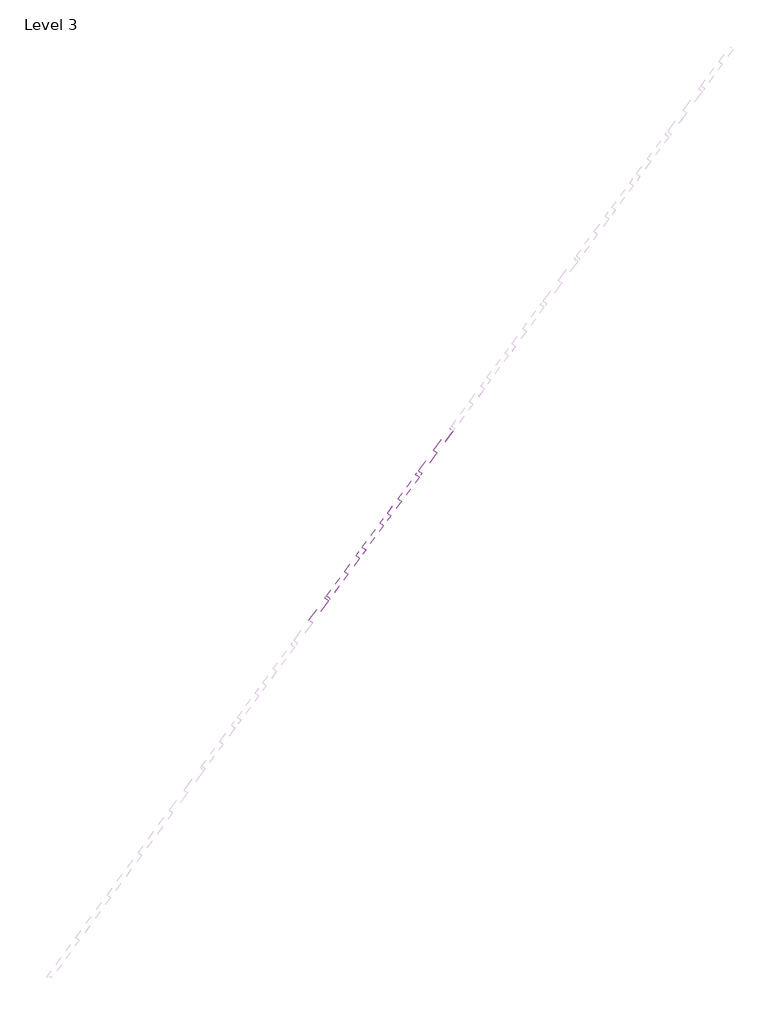
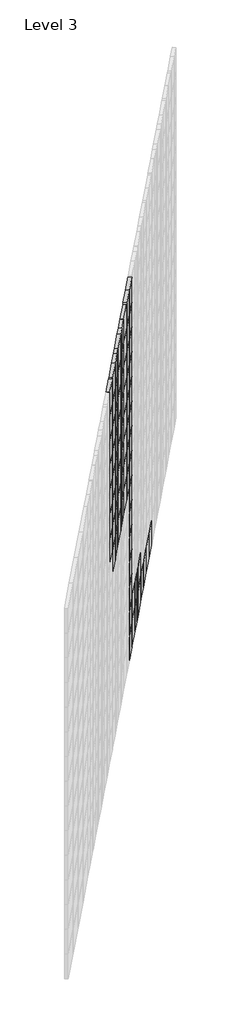
# One storey, part 6 of 9: 117 plates.
"""IFC4 building model written with IfcOpenShell, lengths in millimetres."""

import ifcopenshell
import ifcopenshell.guid

model = None  # the IFC model being written
_history = None  # IfcOwnerHistory: only IFC2X3 demands one
_inside = {}  # id of a spatial element -> (the spatial element, [elements in it])
_under = {}  # id of a project, library or spatial element -> (it, [spatial elements below it])
_declared = {}  # id of a project -> (the project, [libraries it declares])
_typed = {}  # id of a type object -> (the type object, [elements of that type])
_made_of = {}  # id of a material, layer set ... -> (it, [elements and type objects made of it])


def new_model(schema):
    """Start an empty IFC model of exactly this schema.

    Asked for "IFC4X3", IfcOpenShell would pick the latest addendum, in which some entities
    have other attributes; the version numbers below select the first issue.
    IFC2X3 requires an IfcOwnerHistory on every rooted entity: one is made here for all.
    """
    global model, _history
    if schema == "IFC4X3":
        model = ifcopenshell.file(schema_version=(4, 3, 0, 0))
    else:
        model = ifcopenshell.file(schema=schema)
    _inside.clear()
    _under.clear()
    _declared.clear()
    _typed.clear()
    _made_of.clear()
    _history = None
    if model.schema == "IFC2X3":
        org = make("IfcOrganization", Name="unknown")
        user = make(
            "IfcPersonAndOrganization",
            ThePerson=make("IfcPerson", FamilyName="unknown"),
            TheOrganization=org,
        )
        app = make(
            "IfcApplication",
            ApplicationDeveloper=org,
            Version="unknown",
            ApplicationFullName="unknown",
            ApplicationIdentifier="unknown",
        )
        _history = make(
            "IfcOwnerHistory",
            OwningUser=user,
            OwningApplication=app,
            ChangeAction="ADDED",
            CreationDate=0,
        )
    return model


def make(cls, **values):
    """One entity of the class cls with the attributes given. An attribute that is None is left unset."""
    return model.create_entity(
        cls, **{name: value for name, value in values.items() if value is not None}
    )


def rooted(cls, **values):
    """An entity with a GlobalId (a new one), such as an element, a storey or a relation."""
    return make(cls, GlobalId=ifcopenshell.guid.new(), OwnerHistory=_history, **values)


def si_unit(unit_type, name, prefix=None):
    """IfcSIUnit, for example si_unit("LENGTHUNIT", "METRE", prefix="MILLI")."""
    return make("IfcSIUnit", UnitType=unit_type, Prefix=prefix, Name=name)


def assignment(units):
    """IfcUnitAssignment: the units of a project."""
    return None if units is None else make("IfcUnitAssignment", Units=units)


def point(xyz):
    """IfcCartesianPoint."""
    return None if xyz is None else make("IfcCartesianPoint", Coordinates=xyz)


def direction(xyz):
    """IfcDirection."""
    return None if xyz is None else make("IfcDirection", DirectionRatios=xyz)


def frame(location, z_axis=None, x_axis=None):
    """IfcAxis2Placement3D, a coordinate frame: its origin and axes. An axis left out is left unset."""
    return make(
        "IfcAxis2Placement3D",
        Location=point(location),
        Axis=direction(z_axis),
        RefDirection=direction(x_axis),
    )


def origin():
    """The frame at (0, 0, 0) with its axes left unset."""
    return frame((0.0, 0.0, 0.0))


def origin_with_axes():
    """The frame at (0, 0, 0) with the z axis (0, 0, 1) and the x axis (1, 0, 0) written out."""
    return frame((0.0, 0.0, 0.0), z_axis=(0.0, 0.0, 1.0), x_axis=(1.0, 0.0, 0.0))


def place(relative_to, where):
    """IfcLocalPlacement: puts the frame where relative to a parent placement (None: the world)."""
    return make(
        "IfcLocalPlacement", PlacementRelTo=relative_to, RelativePlacement=where
    )


def context(
    kind, dimensions, precision=None, world=None, true_north=None, identifier=None
):
    """IfcGeometricRepresentationContext, for example the 3D "Model" context."""
    return make(
        "IfcGeometricRepresentationContext",
        ContextIdentifier=identifier,
        ContextType=kind,
        CoordinateSpaceDimension=dimensions,
        Precision=precision,
        WorldCoordinateSystem=world,
        TrueNorth=true_north,
    )


def project(units=None, contexts=None):
    """IfcProject with its units and contexts."""
    return rooted(
        "IfcProject",
        Name="project",
        RepresentationContexts=contexts,
        UnitsInContext=assignment(units),
    )


def spatial(cls, under=None, at=None, **own):
    """A site, building, storey or space (cls), placed at a placement, below another one or the project."""
    s = rooted(cls, ObjectPlacement=at, **own)
    if under is not None:
        _under.setdefault(under.id(), (under, []))[1].append(s)
    return s


def polyline(points):
    """IfcPolyline through the points."""
    return make("IfcPolyline", Points=[point(p) for p in points])


def outline(outer, holes=None, kind="AREA"):
    """IfcArbitraryClosedProfileDef: a profile drawn as a closed curve; with holes, ...WithVoids."""
    if holes is None:
        return make("IfcArbitraryClosedProfileDef", ProfileType=kind, OuterCurve=outer)
    return make(
        "IfcArbitraryProfileDefWithVoids",
        ProfileType=kind,
        OuterCurve=outer,
        InnerCurves=holes,
    )


def extrude(swept, where, along, depth):
    """IfcExtrudedAreaSolid: the profile swept, set in the frame where, extruded along a direction by depth."""
    return make(
        "IfcExtrudedAreaSolid",
        SweptArea=swept,
        Position=where,
        ExtrudedDirection=direction(along),
        Depth=depth,
    )


def shape(context_of_items, identifier, shape_type, items):
    """IfcShapeRepresentation: the items that make up one representation, for example the "Body"."""
    return make(
        "IfcShapeRepresentation",
        ContextOfItems=context_of_items,
        RepresentationIdentifier=identifier,
        RepresentationType=shape_type,
        Items=items,
    )


def source(mapping_origin, context_of_items, identifier, shape_type, items):
    """IfcRepresentationMap: a shape defined once, which mapped items show again and again."""
    return make(
        "IfcRepresentationMap",
        MappingOrigin=mapping_origin,
        MappedRepresentation=shape(context_of_items, identifier, shape_type, items),
    )


def transform(
    local_origin,
    x_axis=None,
    y_axis=None,
    z_axis=None,
    scale=None,
    scale2=None,
    scale3=None,
    uniform=True,
):
    """IfcCartesianTransformationOperator3D, or its non-uniform kind. x_axis, y_axis, z_axis: its Axis1, 2, 3."""
    if uniform:
        return make(
            "IfcCartesianTransformationOperator3D",
            Axis1=direction(x_axis),
            Axis2=direction(y_axis),
            LocalOrigin=point(local_origin),
            Scale=scale,
            Axis3=direction(z_axis),
        )
    return make(
        "IfcCartesianTransformationOperator3DnonUniform",
        Axis1=direction(x_axis),
        Axis2=direction(y_axis),
        LocalOrigin=point(local_origin),
        Scale=scale,
        Axis3=direction(z_axis),
        Scale2=scale2,
        Scale3=scale3,
    )


def mapped(mapping_source, mapping_target):
    """IfcMappedItem: shows the shape of a source again, moved by a transform."""
    return make(
        "IfcMappedItem", MappingSource=mapping_source, MappingTarget=mapping_target
    )


def made_of(thing, what):
    """Note that an element or type object is made of a material, layer set ...; save() writes the relation."""
    if what is not None:
        _made_of.setdefault(what.id(), (what, []))[1].append(thing)
    return thing


def element(
    cls,
    number,
    at=None,
    inside=None,
    cuts=None,
    type_object=None,
    material=None,
    context=None,
    identifier="Body",
    shape_type=None,
    held_by="IfcProductDefinitionShape",
    body=None,
    shapes=None,
    **own,
):
    """One element of the class cls, such as IfcWall. Its Tag is "e" and its number.

    at: its placement. inside: the storey or other place that contains it. cuts: it is an
    opening in that element (IfcRelVoidsElement). A single representation is given by context,
    identifier, shape_type and body (its items); several are given by shapes. held_by: the class
    of the entity that holds the representations. save() writes the other relations.
    """
    e = rooted(cls, Tag="e%d" % number, ObjectPlacement=at, **own)
    if body is not None:
        shapes = [shape(context, identifier, shape_type, body)]
    if shapes is not None:
        e.Representation = make(held_by, Representations=shapes)
    if inside is not None:
        _inside.setdefault(inside.id(), (inside, []))[1].append(e)
    if cuts is not None:
        rooted(
            "IfcRelVoidsElement", RelatingBuildingElement=cuts, RelatedOpeningElement=e
        )
    if type_object is not None:
        _typed.setdefault(type_object.id(), (type_object, []))[1].append(e)
    return made_of(e, material)


def aggregate(whole, parts):
    """IfcRelAggregates: a whole, such as a stair, and the parts it consists of."""
    return rooted("IfcRelAggregates", RelatingObject=whole, RelatedObjects=parts)


def save(model, path):
    """Write the relations noted so far, then the file.

    IfcRelAggregates (storeys below a building ...), IfcRelContainedInSpatialStructure (elements
    in a storey), IfcRelDefinesByType, IfcRelAssociatesMaterial and IfcRelDeclares: one each for
    every whole, place, type object, material and project.
    """
    for whole, parts in _under.values():
        aggregate(whole, parts)
    for where, things in _inside.values():
        rooted(
            "IfcRelContainedInSpatialStructure",
            RelatedElements=things,
            RelatingStructure=where,
        )
    for kind, things in _typed.values():
        rooted("IfcRelDefinesByType", RelatedObjects=things, RelatingType=kind)
    for what, things in _made_of.values():
        rooted("IfcRelAssociatesMaterial", RelatedObjects=things, RelatingMaterial=what)
    for by, libraries in _declared.values():
        rooted("IfcRelDeclares", RelatingContext=by, RelatedDefinitions=libraries)
    model.write(path)


def system_panel_glazed_3bc540b8(model_context):
    return source(origin(), model_context, "Body", "SweptSolid", [
        extrude(outline(polyline([(7.4693035, 24.5), (-7.4693035, 24.5), (-7.4693035, 49.5), (7.4693035, 49.5), (7.4693035, 24.5)])), origin_with_axes(), (0.0, 0.0, 1.0), 200.0),
    ])


def system_panel_glazed_0948c99b(model_context):
    return source(origin(), model_context, "Body", "SweptSolid", [
        extrude(outline(polyline([(28.9860643, 24.5), (-28.9860643, 24.5), (-28.9860643, 49.5), (28.9860643, 49.5), (28.9860643, 24.5)])), origin_with_axes(), (0.0, 0.0, 1.0), 200.0),
    ])


def system_panel_glazed_b9ee7cbb(model_context):
    return source(origin(), model_context, "Body", "SweptSolid", [
        extrude(outline(polyline([(50.5028251, 24.5), (-50.5028251, 24.5), (-50.5028251, 49.5), (50.5028251, 49.5), (50.5028251, 24.5)])), origin_with_axes(), (0.0, 0.0, 1.0), 200.0),
    ])


def system_panel_glazed_192fb397(model_context):
    return source(origin(), model_context, "Body", "SweptSolid", [
        extrude(outline(polyline([(72.019586, 24.5), (-72.019586, 24.5), (-72.019586, 49.5), (72.019586, 49.5), (72.019586, 24.5)])), origin_with_axes(), (0.0, 0.0, 1.0), 200.0),
    ])


def system_panel_glazed_b646d57f(model_context):
    return source(origin(), model_context, "Body", "SweptSolid", [
        extrude(outline(polyline([(8.5363468, 24.5), (-8.5363468, 24.5), (-8.5363468, 49.5), (8.5363468, 49.5), (8.5363468, 24.5)])), origin_with_axes(), (0.0, 0.0, 1.0), 200.0),
    ])


def system_panel_glazed_944c5575(model_context):
    return source(origin(), model_context, "Body", "SweptSolid", [
        extrude(outline(polyline([(30.0531077, 24.5), (-30.0531077, 24.5), (-30.0531077, 49.5), (30.0531077, 49.5), (30.0531077, 24.5)])), origin_with_axes(), (0.0, 0.0, 1.0), 200.0),
    ])


def system_panel_glazed_4b393385(model_context):
    return source(origin(), model_context, "Body", "SweptSolid", [
        extrude(outline(polyline([(51.5698685, 24.5), (-51.5698685, 24.5), (-51.5698685, 49.5), (51.5698685, 49.5), (51.5698685, 24.5)])), origin_with_axes(), (0.0, 0.0, 1.0), 200.0),
    ])


def system_panel_glazed_44cc28f0(model_context):
    return source(origin(), model_context, "Body", "SweptSolid", [
        extrude(outline(polyline([(73.0866293, 24.5), (-73.0866293, 24.5), (-73.0866293, 49.5), (73.0866293, 49.5), (73.0866293, 24.5)])), origin_with_axes(), (0.0, 0.0, 1.0), 200.0),
    ])


def system_panel_glazed_1ea8d406(model_context):
    return source(origin(), model_context, "Body", "SweptSolid", [
        extrude(outline(polyline([(85.0, 24.5), (-85.0, 24.5), (-85.0, 49.5), (85.0, 49.5), (85.0, 24.5)])), origin_with_axes(), (0.0, 0.0, 1.0), 200.0),
    ])


def system_panel_glazed_83ffeb2f(model_context):
    return source(origin(), model_context, "Body", "SweptSolid", [
        extrude(outline(polyline([(77.5306965, 24.5), (-77.5306965, 24.5), (-77.5306965, 49.5), (77.5306965, 49.5), (77.5306965, 24.5)])), origin_with_axes(), (0.0, 0.0, 1.0), 200.0),
    ])


def system_panel_glazed_1aaa8be2(model_context):
    return source(origin(), model_context, "Body", "SweptSolid", [
        extrude(outline(polyline([(56.0139357, 24.5), (-56.0139357, 24.5), (-56.0139357, 49.5), (56.0139357, 49.5), (56.0139357, 24.5)])), origin_with_axes(), (0.0, 0.0, 1.0), 200.0),
    ])


def system_panel_glazed_efe9a4c3(model_context):
    return source(origin(), model_context, "Body", "SweptSolid", [
        extrude(outline(polyline([(34.4971749, 24.5), (-34.4971749, 24.5), (-34.4971749, 49.5), (34.4971749, 49.5), (34.4971749, 24.5)])), origin_with_axes(), (0.0, 0.0, 1.0), 200.0),
    ])


def system_panel_glazed_b8c9dfa1(model_context):
    return source(origin(), model_context, "Body", "SweptSolid", [
        extrude(outline(polyline([(12.980414, 24.5), (-12.980414, 24.5), (-12.980414, 49.5), (12.980414, 49.5), (12.980414, 24.5)])), origin_with_axes(), (0.0, 0.0, 1.0), 200.0),
    ])


def system_panel_glazed_2f597917(model_context):
    return source(origin(), model_context, "Body", "SweptSolid", [
        extrude(outline(polyline([(76.4636532, 24.5), (-76.4636532, 24.5), (-76.4636532, 49.5), (76.4636532, 49.5), (76.4636532, 24.5)])), origin_with_axes(), (0.0, 0.0, 1.0), 200.0),
    ])


def system_panel_glazed_a6cffc9f(model_context):
    return source(origin(), model_context, "Body", "SweptSolid", [
        extrude(outline(polyline([(54.9468923, 24.5), (-54.9468923, 24.5), (-54.9468923, 49.5), (54.9468923, 49.5), (54.9468923, 24.5)])), origin_with_axes(), (0.0, 0.0, 1.0), 200.0),
    ])


def system_panel_glazed_52e3984b(model_context):
    return source(origin(), model_context, "Body", "SweptSolid", [
        extrude(outline(polyline([(33.4301315, 24.5), (-33.4301315, 24.5), (-33.4301315, 49.5), (33.4301315, 49.5), (33.4301315, 24.5)])), origin_with_axes(), (0.0, 0.0, 1.0), 200.0),
    ])


def system_panel_glazed_aeb916ba(model_context):
    return source(origin(), model_context, "Body", "SweptSolid", [
        extrude(outline(polyline([(11.9133707, 24.5), (-11.9133707, 24.5), (-11.9133707, 49.5), (11.9133707, 49.5), (11.9133707, 24.5)])), origin_with_axes(), (0.0, 0.0, 1.0), 200.0),
    ])


def system_panel_glazed_a3c9f580(model_context):
    return source(origin(), model_context, "Body", "SweptSolid", [
        extrude(outline(polyline([(75.3966098, 24.5), (-75.3966098, 24.5), (-75.3966098, 49.5), (75.3966098, 49.5), (75.3966098, 24.5)])), origin_with_axes(), (0.0, 0.0, 1.0), 200.0),
    ])


model = new_model("IFC4")

# Units and contexts
model_context = context("Model", 3, world=origin())
ifc_project = project(units=[si_unit("LENGTHUNIT", "METRE", prefix="MILLI")], contexts=[model_context])

# Site, building, storey
site = spatial("IfcSite", under=ifc_project)
building = spatial("IfcBuilding", under=site)
storey = spatial("IfcBuildingStorey", under=building, Name="Level 3", Elevation=22950.0)

# Plates
placement = place(None, origin())
system_panel_glazed_shape = system_panel_glazed_3bc540b8(model_context)
element("IfcPlate", 1, ObjectType="System Panel : Glazed", at=placement, inside=storey, context=model_context, shape_type="MappedRepresentation", body=[
    mapped(system_panel_glazed_shape, transform((-32576.8790424, 29110.0160968, 36700.0), x_axis=(0.5920548138930122, 0.8058976965757569, 0.0), y_axis=(-0.8058976965757569, 0.5920548138930122, 0.0), z_axis=(0.0, 0.0, 1.0))),
])
element("IfcPlate", 2, ObjectType="System Panel : Glazed", at=placement, inside=storey, context=model_context, shape_type="MappedRepresentation", body=[
    mapped(system_panel_glazed_shape, transform((-32576.8790424, 29110.0160968, 36900.0), x_axis=(0.5920548138930122, 0.8058976965757569, 0.0), y_axis=(-0.8058976965757569, 0.5920548138930122, 0.0), z_axis=(0.0, 0.0, 1.0))),
])
element("IfcPlate", 3, ObjectType="System Panel : Glazed", at=placement, inside=storey, context=model_context, shape_type="MappedRepresentation", body=[
    mapped(system_panel_glazed_shape, transform((-32576.8790424, 29110.0160968, 37100.0), x_axis=(0.5920548138930122, 0.8058976965757569, 0.0), y_axis=(-0.8058976965757569, 0.5920548138930122, 0.0), z_axis=(0.0, 0.0, 1.0))),
])
element("IfcPlate", 4, ObjectType="System Panel : Glazed", at=placement, inside=storey, context=model_context, shape_type="MappedRepresentation", body=[
    mapped(system_panel_glazed_shape, transform((-32576.8790424, 29110.0160968, 37300.0), x_axis=(0.5920548138930122, 0.8058976965757569, 0.0), y_axis=(-0.8058976965757569, 0.5920548138930122, 0.0), z_axis=(0.0, 0.0, 1.0))),
])
element("IfcPlate", 5, ObjectType="System Panel : Glazed", at=placement, inside=storey, context=model_context, shape_type="MappedRepresentation", body=[
    mapped(system_panel_glazed_shape, transform((-32576.8790424, 29110.0160968, 37500.0), x_axis=(0.5920548138930122, 0.8058976965757569, 0.0), y_axis=(-0.8058976965757569, 0.5920548138930122, 0.0), z_axis=(0.0, 0.0, 1.0))),
])
element("IfcPlate", 6, ObjectType="System Panel : Glazed", at=placement, inside=storey, context=model_context, shape_type="MappedRepresentation", body=[
    mapped(system_panel_glazed_shape, transform((-32576.8790424, 29110.0160968, 37700.0), x_axis=(0.5920548138930122, 0.8058976965757569, 0.0), y_axis=(-0.8058976965757569, 0.5920548138930122, 0.0), z_axis=(0.0, 0.0, 1.0))),
])
element("IfcPlate", 7, ObjectType="System Panel : Glazed", at=placement, inside=storey, context=model_context, shape_type="MappedRepresentation", body=[
    mapped(system_panel_glazed_shape, transform((-32576.8790424, 29110.0160968, 37900.0), x_axis=(0.5920548138930122, 0.8058976965757569, 0.0), y_axis=(-0.8058976965757569, 0.5920548138930122, 0.0), z_axis=(0.0, 0.0, 1.0))),
])
system_panel_glazed_2_shape = system_panel_glazed_0948c99b(model_context)
element("IfcPlate", 8, ObjectType="System Panel : Glazed", at=placement, inside=storey, context=model_context, shape_type="MappedRepresentation", body=[
    mapped(system_panel_glazed_2_shape, transform((-32388.3195075, 29366.6810057, 36500.0), x_axis=(0.5920548138930122, 0.8058976965757569, 0.0), y_axis=(-0.8058976965757569, 0.5920548138930122, 0.0), z_axis=(0.0, 0.0, 1.0))),
])
element("IfcPlate", 9, ObjectType="System Panel : Glazed", at=placement, inside=storey, context=model_context, shape_type="MappedRepresentation", body=[
    mapped(system_panel_glazed_2_shape, transform((-32388.3195075, 29366.6810057, 36700.0), x_axis=(0.5920548138930122, 0.8058976965757569, 0.0), y_axis=(-0.8058976965757569, 0.5920548138930122, 0.0), z_axis=(0.0, 0.0, 1.0))),
])
element("IfcPlate", 10, ObjectType="System Panel : Glazed", at=placement, inside=storey, context=model_context, shape_type="MappedRepresentation", body=[
    mapped(system_panel_glazed_2_shape, transform((-32388.3195075, 29366.6810057, 36900.0), x_axis=(0.5920548138930122, 0.8058976965757569, 0.0), y_axis=(-0.8058976965757569, 0.5920548138930122, 0.0), z_axis=(0.0, 0.0, 1.0))),
])
element("IfcPlate", 11, ObjectType="System Panel : Glazed", at=placement, inside=storey, context=model_context, shape_type="MappedRepresentation", body=[
    mapped(system_panel_glazed_2_shape, transform((-32388.3195075, 29366.6810057, 37100.0), x_axis=(0.5920548138930122, 0.8058976965757569, 0.0), y_axis=(-0.8058976965757569, 0.5920548138930122, 0.0), z_axis=(0.0, 0.0, 1.0))),
])
element("IfcPlate", 12, ObjectType="System Panel : Glazed", at=placement, inside=storey, context=model_context, shape_type="MappedRepresentation", body=[
    mapped(system_panel_glazed_2_shape, transform((-32388.3195075, 29366.6810057, 37300.0), x_axis=(0.5920548138930122, 0.8058976965757569, 0.0), y_axis=(-0.8058976965757569, 0.5920548138930122, 0.0), z_axis=(0.0, 0.0, 1.0))),
])
element("IfcPlate", 13, ObjectType="System Panel : Glazed", at=placement, inside=storey, context=model_context, shape_type="MappedRepresentation", body=[
    mapped(system_panel_glazed_2_shape, transform((-32388.3195075, 29366.6810057, 37500.0), x_axis=(0.5920548138930122, 0.8058976965757569, 0.0), y_axis=(-0.8058976965757569, 0.5920548138930122, 0.0), z_axis=(0.0, 0.0, 1.0))),
])
element("IfcPlate", 14, ObjectType="System Panel : Glazed", at=placement, inside=storey, context=model_context, shape_type="MappedRepresentation", body=[
    mapped(system_panel_glazed_2_shape, transform((-32388.3195075, 29366.6810057, 37700.0), x_axis=(0.5920548138930122, 0.8058976965757569, 0.0), y_axis=(-0.8058976965757569, 0.5920548138930122, 0.0), z_axis=(0.0, 0.0, 1.0))),
])
element("IfcPlate", 15, ObjectType="System Panel : Glazed", at=placement, inside=storey, context=model_context, shape_type="MappedRepresentation", body=[
    mapped(system_panel_glazed_2_shape, transform((-32388.3195075, 29366.6810057, 37900.0), x_axis=(0.5920548138930122, 0.8058976965757569, 0.0), y_axis=(-0.8058976965757569, 0.5920548138930122, 0.0), z_axis=(0.0, 0.0, 1.0))),
])
system_panel_glazed_3_shape = system_panel_glazed_b9ee7cbb(model_context)
element("IfcPlate", 16, ObjectType="System Panel : Glazed", at=placement, inside=storey, context=model_context, shape_type="MappedRepresentation", body=[
    mapped(system_panel_glazed_3_shape, transform((-32199.7599726, 29623.3459145, 36500.0), x_axis=(0.5920548138930122, 0.8058976965757569, 0.0), y_axis=(-0.8058976965757569, 0.5920548138930122, 0.0), z_axis=(0.0, 0.0, 1.0))),
])
element("IfcPlate", 17, ObjectType="System Panel : Glazed", at=placement, inside=storey, context=model_context, shape_type="MappedRepresentation", body=[
    mapped(system_panel_glazed_3_shape, transform((-32199.7599726, 29623.3459145, 36700.0), x_axis=(0.5920548138930122, 0.8058976965757569, 0.0), y_axis=(-0.8058976965757569, 0.5920548138930122, 0.0), z_axis=(0.0, 0.0, 1.0))),
])
element("IfcPlate", 18, ObjectType="System Panel : Glazed", at=placement, inside=storey, context=model_context, shape_type="MappedRepresentation", body=[
    mapped(system_panel_glazed_3_shape, transform((-32199.7599726, 29623.3459145, 36900.0), x_axis=(0.5920548138930122, 0.8058976965757569, 0.0), y_axis=(-0.8058976965757569, 0.5920548138930122, 0.0), z_axis=(0.0, 0.0, 1.0))),
])
element("IfcPlate", 19, ObjectType="System Panel : Glazed", at=placement, inside=storey, context=model_context, shape_type="MappedRepresentation", body=[
    mapped(system_panel_glazed_3_shape, transform((-32199.7599726, 29623.3459145, 37100.0), x_axis=(0.5920548138930122, 0.8058976965757569, 0.0), y_axis=(-0.8058976965757569, 0.5920548138930122, 0.0), z_axis=(0.0, 0.0, 1.0))),
])
element("IfcPlate", 20, ObjectType="System Panel : Glazed", at=placement, inside=storey, context=model_context, shape_type="MappedRepresentation", body=[
    mapped(system_panel_glazed_3_shape, transform((-32199.7599726, 29623.3459145, 37300.0), x_axis=(0.5920548138930122, 0.8058976965757569, 0.0), y_axis=(-0.8058976965757569, 0.5920548138930122, 0.0), z_axis=(0.0, 0.0, 1.0))),
])
element("IfcPlate", 21, ObjectType="System Panel : Glazed", at=placement, inside=storey, context=model_context, shape_type="MappedRepresentation", body=[
    mapped(system_panel_glazed_3_shape, transform((-32199.7599726, 29623.3459145, 37500.0), x_axis=(0.5920548138930122, 0.8058976965757569, 0.0), y_axis=(-0.8058976965757569, 0.5920548138930122, 0.0), z_axis=(0.0, 0.0, 1.0))),
])
element("IfcPlate", 22, ObjectType="System Panel : Glazed", at=placement, inside=storey, context=model_context, shape_type="MappedRepresentation", body=[
    mapped(system_panel_glazed_3_shape, transform((-32199.7599726, 29623.3459145, 37700.0), x_axis=(0.5920548138930122, 0.8058976965757569, 0.0), y_axis=(-0.8058976965757569, 0.5920548138930122, 0.0), z_axis=(0.0, 0.0, 1.0))),
])
element("IfcPlate", 23, ObjectType="System Panel : Glazed", at=placement, inside=storey, context=model_context, shape_type="MappedRepresentation", body=[
    mapped(system_panel_glazed_3_shape, transform((-32199.7599726, 29623.3459145, 37900.0), x_axis=(0.5920548138930122, 0.8058976965757569, 0.0), y_axis=(-0.8058976965757569, 0.5920548138930122, 0.0), z_axis=(0.0, 0.0, 1.0))),
])
system_panel_glazed_4_shape = system_panel_glazed_192fb397(model_context)
element("IfcPlate", 24, ObjectType="System Panel : Glazed", at=placement, inside=storey, context=model_context, shape_type="MappedRepresentation", body=[
    mapped(system_panel_glazed_4_shape, transform((-32011.2004377, 29880.0108233, 36500.0), x_axis=(0.5920548138930122, 0.8058976965757569, 0.0), y_axis=(-0.8058976965757569, 0.5920548138930122, 0.0), z_axis=(0.0, 0.0, 1.0))),
])
element("IfcPlate", 25, ObjectType="System Panel : Glazed", at=placement, inside=storey, context=model_context, shape_type="MappedRepresentation", body=[
    mapped(system_panel_glazed_4_shape, transform((-32011.2004377, 29880.0108233, 36700.0), x_axis=(0.5920548138930122, 0.8058976965757569, 0.0), y_axis=(-0.8058976965757569, 0.5920548138930122, 0.0), z_axis=(0.0, 0.0, 1.0))),
])
element("IfcPlate", 26, ObjectType="System Panel : Glazed", at=placement, inside=storey, context=model_context, shape_type="MappedRepresentation", body=[
    mapped(system_panel_glazed_4_shape, transform((-32011.2004377, 29880.0108233, 36900.0), x_axis=(0.5920548138930122, 0.8058976965757569, 0.0), y_axis=(-0.8058976965757569, 0.5920548138930122, 0.0), z_axis=(0.0, 0.0, 1.0))),
])
element("IfcPlate", 27, ObjectType="System Panel : Glazed", at=placement, inside=storey, context=model_context, shape_type="MappedRepresentation", body=[
    mapped(system_panel_glazed_4_shape, transform((-32011.2004377, 29880.0108233, 37100.0), x_axis=(0.5920548138930122, 0.8058976965757569, 0.0), y_axis=(-0.8058976965757569, 0.5920548138930122, 0.0), z_axis=(0.0, 0.0, 1.0))),
])
element("IfcPlate", 28, ObjectType="System Panel : Glazed", at=placement, inside=storey, context=model_context, shape_type="MappedRepresentation", body=[
    mapped(system_panel_glazed_4_shape, transform((-32011.2004377, 29880.0108233, 37300.0), x_axis=(0.5920548138930122, 0.8058976965757569, 0.0), y_axis=(-0.8058976965757569, 0.5920548138930122, 0.0), z_axis=(0.0, 0.0, 1.0))),
])
element("IfcPlate", 29, ObjectType="System Panel : Glazed", at=placement, inside=storey, context=model_context, shape_type="MappedRepresentation", body=[
    mapped(system_panel_glazed_4_shape, transform((-32011.2004377, 29880.0108233, 37500.0), x_axis=(0.5920548138930122, 0.8058976965757569, 0.0), y_axis=(-0.8058976965757569, 0.5920548138930122, 0.0), z_axis=(0.0, 0.0, 1.0))),
])
element("IfcPlate", 30, ObjectType="System Panel : Glazed", at=placement, inside=storey, context=model_context, shape_type="MappedRepresentation", body=[
    mapped(system_panel_glazed_4_shape, transform((-32011.2004377, 29880.0108233, 37700.0), x_axis=(0.5920548138930122, 0.8058976965757569, 0.0), y_axis=(-0.8058976965757569, 0.5920548138930122, 0.0), z_axis=(0.0, 0.0, 1.0))),
])
element("IfcPlate", 31, ObjectType="System Panel : Glazed", at=placement, inside=storey, context=model_context, shape_type="MappedRepresentation", body=[
    mapped(system_panel_glazed_4_shape, transform((-32011.2004377, 29880.0108233, 37900.0), x_axis=(0.5920548138930122, 0.8058976965757569, 0.0), y_axis=(-0.8058976965757569, 0.5920548138930122, 0.0), z_axis=(0.0, 0.0, 1.0))),
])
system_panel_glazed_5_shape = system_panel_glazed_b646d57f(model_context)
element("IfcPlate", 32, ObjectType="System Panel : Glazed", at=placement, inside=storey, context=model_context, shape_type="MappedRepresentation", body=[
    mapped(system_panel_glazed_5_shape, transform((-31872.965562, 30068.174428, 35100.0), x_axis=(0.5920548138930122, 0.8058976965757569, 0.0), y_axis=(-0.8058976965757569, 0.5920548138930122, 0.0), z_axis=(0.0, 0.0, 1.0))),
])
element("IfcPlate", 33, ObjectType="System Panel : Glazed", at=placement, inside=storey, context=model_context, shape_type="MappedRepresentation", body=[
    mapped(system_panel_glazed_5_shape, transform((-31872.965562, 30068.174428, 35300.0), x_axis=(0.5920548138930122, 0.8058976965757569, 0.0), y_axis=(-0.8058976965757569, 0.5920548138930122, 0.0), z_axis=(0.0, 0.0, 1.0))),
])
system_panel_glazed_6_shape = system_panel_glazed_944c5575(model_context)
element("IfcPlate", 34, ObjectType="System Panel : Glazed", at=placement, inside=storey, context=model_context, shape_type="MappedRepresentation", body=[
    mapped(system_panel_glazed_6_shape, transform((-31684.4060271, 30324.8393368, 35100.0), x_axis=(0.5920548138930122, 0.8058976965757569, 0.0), y_axis=(-0.8058976965757569, 0.5920548138930122, 0.0), z_axis=(0.0, 0.0, 1.0))),
])
element("IfcPlate", 35, ObjectType="System Panel : Glazed", at=placement, inside=storey, context=model_context, shape_type="MappedRepresentation", body=[
    mapped(system_panel_glazed_6_shape, transform((-31684.4060271, 30324.8393368, 35300.0), x_axis=(0.5920548138930122, 0.8058976965757569, 0.0), y_axis=(-0.8058976965757569, 0.5920548138930122, 0.0), z_axis=(0.0, 0.0, 1.0))),
])
system_panel_glazed_7_shape = system_panel_glazed_4b393385(model_context)
element("IfcPlate", 36, ObjectType="System Panel : Glazed", at=placement, inside=storey, context=model_context, shape_type="MappedRepresentation", body=[
    mapped(system_panel_glazed_7_shape, transform((-31495.8464922, 30581.5042456, 35100.0), x_axis=(0.5920548138930122, 0.8058976965757569, 0.0), y_axis=(-0.8058976965757569, 0.5920548138930122, 0.0), z_axis=(0.0, 0.0, 1.0))),
])
system_panel_glazed_8_shape = system_panel_glazed_44cc28f0(model_context)
element("IfcPlate", 37, ObjectType="System Panel : Glazed", at=placement, inside=storey, context=model_context, shape_type="MappedRepresentation", body=[
    mapped(system_panel_glazed_8_shape, transform((-31307.2869573, 30838.1691545, 35100.0), x_axis=(0.5920548138930122, 0.8058976965757569, 0.0), y_axis=(-0.8058976965757569, 0.5920548138930122, 0.0), z_axis=(0.0, 0.0, 1.0))),
])
system_panel_glazed_9_shape = system_panel_glazed_1ea8d406(model_context)
element("IfcPlate", 38, ObjectType="System Panel : Glazed", at=placement, inside=storey, context=model_context, shape_type="MappedRepresentation", body=[
    mapped(system_panel_glazed_9_shape, transform((-31817.5869176, 30143.5551544, 35100.0), x_axis=(0.5920548138930122, 0.8058976965757569, 0.0), y_axis=(-0.8058976965757569, 0.5920548138930122, 0.0), z_axis=(0.0, 0.0, 1.0))),
])
element("IfcPlate", 39, ObjectType="System Panel : Glazed", at=placement, inside=storey, context=model_context, shape_type="MappedRepresentation", body=[
    mapped(system_panel_glazed_9_shape, transform((-31616.2882809, 30417.5603713, 35100.0), x_axis=(0.5920548138930122, 0.8058976965757569, 0.0), y_axis=(-0.8058976965757569, 0.5920548138930122, 0.0), z_axis=(0.0, 0.0, 1.0))),
])
element("IfcPlate", 40, ObjectType="System Panel : Glazed", at=placement, inside=storey, context=model_context, shape_type="MappedRepresentation", body=[
    mapped(system_panel_glazed_9_shape, transform((-31414.9896441, 30691.5655881, 35100.0), x_axis=(0.5920548138930122, 0.8058976965757569, 0.0), y_axis=(-0.8058976965757569, 0.5920548138930122, 0.0), z_axis=(0.0, 0.0, 1.0))),
])
element("IfcPlate", 41, ObjectType="System Panel : Glazed", at=placement, inside=storey, context=model_context, shape_type="MappedRepresentation", body=[
    mapped(system_panel_glazed_9_shape, transform((-31817.5869176, 30143.5551544, 35300.0), x_axis=(0.5920548138930122, 0.8058976965757569, 0.0), y_axis=(-0.8058976965757569, 0.5920548138930122, 0.0), z_axis=(0.0, 0.0, 1.0))),
])
element("IfcPlate", 42, ObjectType="System Panel : Glazed", at=placement, inside=storey, context=model_context, shape_type="MappedRepresentation", body=[
    mapped(system_panel_glazed_9_shape, transform((-31616.2882809, 30417.5603713, 35300.0), x_axis=(0.5920548138930122, 0.8058976965757569, 0.0), y_axis=(-0.8058976965757569, 0.5920548138930122, 0.0), z_axis=(0.0, 0.0, 1.0))),
])
element("IfcPlate", 43, ObjectType="System Panel : Glazed", at=placement, inside=storey, context=model_context, shape_type="MappedRepresentation", body=[
    mapped(system_panel_glazed_9_shape, transform((-32522.1321461, 29184.5368955, 36500.0), x_axis=(0.5920548138930122, 0.8058976965757569, 0.0), y_axis=(-0.8058976965757569, 0.5920548138930122, 0.0), z_axis=(0.0, 0.0, 1.0))),
])
element("IfcPlate", 44, ObjectType="System Panel : Glazed", at=placement, inside=storey, context=model_context, shape_type="MappedRepresentation", body=[
    mapped(system_panel_glazed_9_shape, transform((-32320.8335094, 29458.5421123, 36500.0), x_axis=(0.5920548138930122, 0.8058976965757569, 0.0), y_axis=(-0.8058976965757569, 0.5920548138930122, 0.0), z_axis=(0.0, 0.0, 1.0))),
])
element("IfcPlate", 45, ObjectType="System Panel : Glazed", at=placement, inside=storey, context=model_context, shape_type="MappedRepresentation", body=[
    mapped(system_panel_glazed_9_shape, transform((-32119.5348727, 29732.5473292, 36500.0), x_axis=(0.5920548138930122, 0.8058976965757569, 0.0), y_axis=(-0.8058976965757569, 0.5920548138930122, 0.0), z_axis=(0.0, 0.0, 1.0))),
])
element("IfcPlate", 46, ObjectType="System Panel : Glazed", at=placement, inside=storey, context=model_context, shape_type="MappedRepresentation", body=[
    mapped(system_panel_glazed_9_shape, transform((-32522.1321461, 29184.5368955, 36700.0), x_axis=(0.5920548138930122, 0.8058976965757569, 0.0), y_axis=(-0.8058976965757569, 0.5920548138930122, 0.0), z_axis=(0.0, 0.0, 1.0))),
])
element("IfcPlate", 47, ObjectType="System Panel : Glazed", at=placement, inside=storey, context=model_context, shape_type="MappedRepresentation", body=[
    mapped(system_panel_glazed_9_shape, transform((-32320.8335094, 29458.5421123, 36700.0), x_axis=(0.5920548138930122, 0.8058976965757569, 0.0), y_axis=(-0.8058976965757569, 0.5920548138930122, 0.0), z_axis=(0.0, 0.0, 1.0))),
])
element("IfcPlate", 48, ObjectType="System Panel : Glazed", at=placement, inside=storey, context=model_context, shape_type="MappedRepresentation", body=[
    mapped(system_panel_glazed_9_shape, transform((-32119.5348727, 29732.5473292, 36700.0), x_axis=(0.5920548138930122, 0.8058976965757569, 0.0), y_axis=(-0.8058976965757569, 0.5920548138930122, 0.0), z_axis=(0.0, 0.0, 1.0))),
])
element("IfcPlate", 49, ObjectType="System Panel : Glazed", at=placement, inside=storey, context=model_context, shape_type="MappedRepresentation", body=[
    mapped(system_panel_glazed_9_shape, transform((-32522.1321461, 29184.5368955, 36900.0), x_axis=(0.5920548138930122, 0.8058976965757569, 0.0), y_axis=(-0.8058976965757569, 0.5920548138930122, 0.0), z_axis=(0.0, 0.0, 1.0))),
])
element("IfcPlate", 50, ObjectType="System Panel : Glazed", at=placement, inside=storey, context=model_context, shape_type="MappedRepresentation", body=[
    mapped(system_panel_glazed_9_shape, transform((-32320.8335094, 29458.5421123, 36900.0), x_axis=(0.5920548138930122, 0.8058976965757569, 0.0), y_axis=(-0.8058976965757569, 0.5920548138930122, 0.0), z_axis=(0.0, 0.0, 1.0))),
])
element("IfcPlate", 51, ObjectType="System Panel : Glazed", at=placement, inside=storey, context=model_context, shape_type="MappedRepresentation", body=[
    mapped(system_panel_glazed_9_shape, transform((-32119.5348727, 29732.5473292, 36900.0), x_axis=(0.5920548138930122, 0.8058976965757569, 0.0), y_axis=(-0.8058976965757569, 0.5920548138930122, 0.0), z_axis=(0.0, 0.0, 1.0))),
])
element("IfcPlate", 52, ObjectType="System Panel : Glazed", at=placement, inside=storey, context=model_context, shape_type="MappedRepresentation", body=[
    mapped(system_panel_glazed_9_shape, transform((-32522.1321461, 29184.5368955, 37100.0), x_axis=(0.5920548138930122, 0.8058976965757569, 0.0), y_axis=(-0.8058976965757569, 0.5920548138930122, 0.0), z_axis=(0.0, 0.0, 1.0))),
])
element("IfcPlate", 53, ObjectType="System Panel : Glazed", at=placement, inside=storey, context=model_context, shape_type="MappedRepresentation", body=[
    mapped(system_panel_glazed_9_shape, transform((-32320.8335094, 29458.5421123, 37100.0), x_axis=(0.5920548138930122, 0.8058976965757569, 0.0), y_axis=(-0.8058976965757569, 0.5920548138930122, 0.0), z_axis=(0.0, 0.0, 1.0))),
])
element("IfcPlate", 54, ObjectType="System Panel : Glazed", at=placement, inside=storey, context=model_context, shape_type="MappedRepresentation", body=[
    mapped(system_panel_glazed_9_shape, transform((-32119.5348727, 29732.5473292, 37100.0), x_axis=(0.5920548138930122, 0.8058976965757569, 0.0), y_axis=(-0.8058976965757569, 0.5920548138930122, 0.0), z_axis=(0.0, 0.0, 1.0))),
])
element("IfcPlate", 55, ObjectType="System Panel : Glazed", at=placement, inside=storey, context=model_context, shape_type="MappedRepresentation", body=[
    mapped(system_panel_glazed_9_shape, transform((-32522.1321461, 29184.5368955, 37300.0), x_axis=(0.5920548138930122, 0.8058976965757569, 0.0), y_axis=(-0.8058976965757569, 0.5920548138930122, 0.0), z_axis=(0.0, 0.0, 1.0))),
])
element("IfcPlate", 56, ObjectType="System Panel : Glazed", at=placement, inside=storey, context=model_context, shape_type="MappedRepresentation", body=[
    mapped(system_panel_glazed_9_shape, transform((-32320.8335094, 29458.5421123, 37300.0), x_axis=(0.5920548138930122, 0.8058976965757569, 0.0), y_axis=(-0.8058976965757569, 0.5920548138930122, 0.0), z_axis=(0.0, 0.0, 1.0))),
])
element("IfcPlate", 57, ObjectType="System Panel : Glazed", at=placement, inside=storey, context=model_context, shape_type="MappedRepresentation", body=[
    mapped(system_panel_glazed_9_shape, transform((-32119.5348727, 29732.5473292, 37300.0), x_axis=(0.5920548138930122, 0.8058976965757569, 0.0), y_axis=(-0.8058976965757569, 0.5920548138930122, 0.0), z_axis=(0.0, 0.0, 1.0))),
])
element("IfcPlate", 58, ObjectType="System Panel : Glazed", at=placement, inside=storey, context=model_context, shape_type="MappedRepresentation", body=[
    mapped(system_panel_glazed_9_shape, transform((-32522.1321461, 29184.5368955, 37500.0), x_axis=(0.5920548138930122, 0.8058976965757569, 0.0), y_axis=(-0.8058976965757569, 0.5920548138930122, 0.0), z_axis=(0.0, 0.0, 1.0))),
])
element("IfcPlate", 59, ObjectType="System Panel : Glazed", at=placement, inside=storey, context=model_context, shape_type="MappedRepresentation", body=[
    mapped(system_panel_glazed_9_shape, transform((-32320.8335094, 29458.5421123, 37500.0), x_axis=(0.5920548138930122, 0.8058976965757569, 0.0), y_axis=(-0.8058976965757569, 0.5920548138930122, 0.0), z_axis=(0.0, 0.0, 1.0))),
])
element("IfcPlate", 60, ObjectType="System Panel : Glazed", at=placement, inside=storey, context=model_context, shape_type="MappedRepresentation", body=[
    mapped(system_panel_glazed_9_shape, transform((-32119.5348727, 29732.5473292, 37500.0), x_axis=(0.5920548138930122, 0.8058976965757569, 0.0), y_axis=(-0.8058976965757569, 0.5920548138930122, 0.0), z_axis=(0.0, 0.0, 1.0))),
])
element("IfcPlate", 61, ObjectType="System Panel : Glazed", at=placement, inside=storey, context=model_context, shape_type="MappedRepresentation", body=[
    mapped(system_panel_glazed_9_shape, transform((-32522.1321461, 29184.5368955, 37700.0), x_axis=(0.5920548138930122, 0.8058976965757569, 0.0), y_axis=(-0.8058976965757569, 0.5920548138930122, 0.0), z_axis=(0.0, 0.0, 1.0))),
])
element("IfcPlate", 62, ObjectType="System Panel : Glazed", at=placement, inside=storey, context=model_context, shape_type="MappedRepresentation", body=[
    mapped(system_panel_glazed_9_shape, transform((-32320.8335094, 29458.5421123, 37700.0), x_axis=(0.5920548138930122, 0.8058976965757569, 0.0), y_axis=(-0.8058976965757569, 0.5920548138930122, 0.0), z_axis=(0.0, 0.0, 1.0))),
])
element("IfcPlate", 63, ObjectType="System Panel : Glazed", at=placement, inside=storey, context=model_context, shape_type="MappedRepresentation", body=[
    mapped(system_panel_glazed_9_shape, transform((-32119.5348727, 29732.5473292, 37700.0), x_axis=(0.5920548138930122, 0.8058976965757569, 0.0), y_axis=(-0.8058976965757569, 0.5920548138930122, 0.0), z_axis=(0.0, 0.0, 1.0))),
])
element("IfcPlate", 64, ObjectType="System Panel : Glazed", at=placement, inside=storey, context=model_context, shape_type="MappedRepresentation", body=[
    mapped(system_panel_glazed_9_shape, transform((-32522.1321461, 29184.5368955, 37900.0), x_axis=(0.5920548138930122, 0.8058976965757569, 0.0), y_axis=(-0.8058976965757569, 0.5920548138930122, 0.0), z_axis=(0.0, 0.0, 1.0))),
])
element("IfcPlate", 65, ObjectType="System Panel : Glazed", at=placement, inside=storey, context=model_context, shape_type="MappedRepresentation", body=[
    mapped(system_panel_glazed_9_shape, transform((-32320.8335094, 29458.5421123, 37900.0), x_axis=(0.5920548138930122, 0.8058976965757569, 0.0), y_axis=(-0.8058976965757569, 0.5920548138930122, 0.0), z_axis=(0.0, 0.0, 1.0))),
])
element("IfcPlate", 66, ObjectType="System Panel : Glazed", at=placement, inside=storey, context=model_context, shape_type="MappedRepresentation", body=[
    mapped(system_panel_glazed_9_shape, transform((-32119.5348727, 29732.5473292, 37900.0), x_axis=(0.5920548138930122, 0.8058976965757569, 0.0), y_axis=(-0.8058976965757569, 0.5920548138930122, 0.0), z_axis=(0.0, 0.0, 1.0))),
])
system_panel_glazed_10_shape = system_panel_glazed_83ffeb2f(model_context)
element("IfcPlate", 67, ObjectType="System Panel : Glazed", at=placement, inside=storey, context=model_context, shape_type="MappedRepresentation", body=[
    mapped(system_panel_glazed_10_shape, transform((-32627.2037016, 29041.5147926, 36700.0), x_axis=(0.5920548138930122, 0.8058976965757569, 0.0), y_axis=(-0.8058976965757569, 0.5920548138930122, 0.0), z_axis=(0.0, 0.0, 1.0))),
])
element("IfcPlate", 68, ObjectType="System Panel : Glazed", at=placement, inside=storey, context=model_context, shape_type="MappedRepresentation", body=[
    mapped(system_panel_glazed_10_shape, transform((-32627.2037016, 29041.5147926, 36900.0), x_axis=(0.5920548138930122, 0.8058976965757569, 0.0), y_axis=(-0.8058976965757569, 0.5920548138930122, 0.0), z_axis=(0.0, 0.0, 1.0))),
])
element("IfcPlate", 69, ObjectType="System Panel : Glazed", at=placement, inside=storey, context=model_context, shape_type="MappedRepresentation", body=[
    mapped(system_panel_glazed_10_shape, transform((-32627.2037016, 29041.5147926, 37100.0), x_axis=(0.5920548138930122, 0.8058976965757569, 0.0), y_axis=(-0.8058976965757569, 0.5920548138930122, 0.0), z_axis=(0.0, 0.0, 1.0))),
])
element("IfcPlate", 70, ObjectType="System Panel : Glazed", at=placement, inside=storey, context=model_context, shape_type="MappedRepresentation", body=[
    mapped(system_panel_glazed_10_shape, transform((-32627.2037016, 29041.5147926, 37300.0), x_axis=(0.5920548138930122, 0.8058976965757569, 0.0), y_axis=(-0.8058976965757569, 0.5920548138930122, 0.0), z_axis=(0.0, 0.0, 1.0))),
])
element("IfcPlate", 71, ObjectType="System Panel : Glazed", at=placement, inside=storey, context=model_context, shape_type="MappedRepresentation", body=[
    mapped(system_panel_glazed_10_shape, transform((-32627.2037016, 29041.5147926, 37500.0), x_axis=(0.5920548138930122, 0.8058976965757569, 0.0), y_axis=(-0.8058976965757569, 0.5920548138930122, 0.0), z_axis=(0.0, 0.0, 1.0))),
])
element("IfcPlate", 72, ObjectType="System Panel : Glazed", at=placement, inside=storey, context=model_context, shape_type="MappedRepresentation", body=[
    mapped(system_panel_glazed_10_shape, transform((-32627.2037016, 29041.5147926, 37700.0), x_axis=(0.5920548138930122, 0.8058976965757569, 0.0), y_axis=(-0.8058976965757569, 0.5920548138930122, 0.0), z_axis=(0.0, 0.0, 1.0))),
])
element("IfcPlate", 73, ObjectType="System Panel : Glazed", at=placement, inside=storey, context=model_context, shape_type="MappedRepresentation", body=[
    mapped(system_panel_glazed_10_shape, transform((-32627.2037016, 29041.5147926, 37900.0), x_axis=(0.5920548138930122, 0.8058976965757569, 0.0), y_axis=(-0.8058976965757569, 0.5920548138930122, 0.0), z_axis=(0.0, 0.0, 1.0))),
])
system_panel_glazed_11_shape = system_panel_glazed_1aaa8be2(model_context)
element("IfcPlate", 74, ObjectType="System Panel : Glazed", at=placement, inside=storey, context=model_context, shape_type="MappedRepresentation", body=[
    mapped(system_panel_glazed_11_shape, transform((-32438.6441667, 29298.1797015, 36500.0), x_axis=(0.5920548138930122, 0.8058976965757569, 0.0), y_axis=(-0.8058976965757569, 0.5920548138930122, 0.0), z_axis=(0.0, 0.0, 1.0))),
])
element("IfcPlate", 75, ObjectType="System Panel : Glazed", at=placement, inside=storey, context=model_context, shape_type="MappedRepresentation", body=[
    mapped(system_panel_glazed_11_shape, transform((-32438.6441667, 29298.1797015, 36700.0), x_axis=(0.5920548138930122, 0.8058976965757569, 0.0), y_axis=(-0.8058976965757569, 0.5920548138930122, 0.0), z_axis=(0.0, 0.0, 1.0))),
])
element("IfcPlate", 76, ObjectType="System Panel : Glazed", at=placement, inside=storey, context=model_context, shape_type="MappedRepresentation", body=[
    mapped(system_panel_glazed_11_shape, transform((-32438.6441667, 29298.1797015, 36900.0), x_axis=(0.5920548138930122, 0.8058976965757569, 0.0), y_axis=(-0.8058976965757569, 0.5920548138930122, 0.0), z_axis=(0.0, 0.0, 1.0))),
])
element("IfcPlate", 77, ObjectType="System Panel : Glazed", at=placement, inside=storey, context=model_context, shape_type="MappedRepresentation", body=[
    mapped(system_panel_glazed_11_shape, transform((-32438.6441667, 29298.1797015, 37100.0), x_axis=(0.5920548138930122, 0.8058976965757569, 0.0), y_axis=(-0.8058976965757569, 0.5920548138930122, 0.0), z_axis=(0.0, 0.0, 1.0))),
])
element("IfcPlate", 78, ObjectType="System Panel : Glazed", at=placement, inside=storey, context=model_context, shape_type="MappedRepresentation", body=[
    mapped(system_panel_glazed_11_shape, transform((-32438.6441667, 29298.1797015, 37300.0), x_axis=(0.5920548138930122, 0.8058976965757569, 0.0), y_axis=(-0.8058976965757569, 0.5920548138930122, 0.0), z_axis=(0.0, 0.0, 1.0))),
])
element("IfcPlate", 79, ObjectType="System Panel : Glazed", at=placement, inside=storey, context=model_context, shape_type="MappedRepresentation", body=[
    mapped(system_panel_glazed_11_shape, transform((-32438.6441667, 29298.1797015, 37500.0), x_axis=(0.5920548138930122, 0.8058976965757569, 0.0), y_axis=(-0.8058976965757569, 0.5920548138930122, 0.0), z_axis=(0.0, 0.0, 1.0))),
])
element("IfcPlate", 80, ObjectType="System Panel : Glazed", at=placement, inside=storey, context=model_context, shape_type="MappedRepresentation", body=[
    mapped(system_panel_glazed_11_shape, transform((-32438.6441667, 29298.1797015, 37700.0), x_axis=(0.5920548138930122, 0.8058976965757569, 0.0), y_axis=(-0.8058976965757569, 0.5920548138930122, 0.0), z_axis=(0.0, 0.0, 1.0))),
])
element("IfcPlate", 81, ObjectType="System Panel : Glazed", at=placement, inside=storey, context=model_context, shape_type="MappedRepresentation", body=[
    mapped(system_panel_glazed_11_shape, transform((-32438.6441667, 29298.1797015, 37900.0), x_axis=(0.5920548138930122, 0.8058976965757569, 0.0), y_axis=(-0.8058976965757569, 0.5920548138930122, 0.0), z_axis=(0.0, 0.0, 1.0))),
])
system_panel_glazed_12_shape = system_panel_glazed_efe9a4c3(model_context)
element("IfcPlate", 82, ObjectType="System Panel : Glazed", at=placement, inside=storey, context=model_context, shape_type="MappedRepresentation", body=[
    mapped(system_panel_glazed_12_shape, transform((-32250.0846318, 29554.8446103, 36500.0), x_axis=(0.5920548138930122, 0.8058976965757569, 0.0), y_axis=(-0.8058976965757569, 0.5920548138930122, 0.0), z_axis=(0.0, 0.0, 1.0))),
])
element("IfcPlate", 83, ObjectType="System Panel : Glazed", at=placement, inside=storey, context=model_context, shape_type="MappedRepresentation", body=[
    mapped(system_panel_glazed_12_shape, transform((-32250.0846318, 29554.8446103, 36700.0), x_axis=(0.5920548138930122, 0.8058976965757569, 0.0), y_axis=(-0.8058976965757569, 0.5920548138930122, 0.0), z_axis=(0.0, 0.0, 1.0))),
])
element("IfcPlate", 84, ObjectType="System Panel : Glazed", at=placement, inside=storey, context=model_context, shape_type="MappedRepresentation", body=[
    mapped(system_panel_glazed_12_shape, transform((-32250.0846318, 29554.8446103, 36900.0), x_axis=(0.5920548138930122, 0.8058976965757569, 0.0), y_axis=(-0.8058976965757569, 0.5920548138930122, 0.0), z_axis=(0.0, 0.0, 1.0))),
])
element("IfcPlate", 85, ObjectType="System Panel : Glazed", at=placement, inside=storey, context=model_context, shape_type="MappedRepresentation", body=[
    mapped(system_panel_glazed_12_shape, transform((-32250.0846318, 29554.8446103, 37100.0), x_axis=(0.5920548138930122, 0.8058976965757569, 0.0), y_axis=(-0.8058976965757569, 0.5920548138930122, 0.0), z_axis=(0.0, 0.0, 1.0))),
])
element("IfcPlate", 86, ObjectType="System Panel : Glazed", at=placement, inside=storey, context=model_context, shape_type="MappedRepresentation", body=[
    mapped(system_panel_glazed_12_shape, transform((-32250.0846318, 29554.8446103, 37300.0), x_axis=(0.5920548138930122, 0.8058976965757569, 0.0), y_axis=(-0.8058976965757569, 0.5920548138930122, 0.0), z_axis=(0.0, 0.0, 1.0))),
])
element("IfcPlate", 87, ObjectType="System Panel : Glazed", at=placement, inside=storey, context=model_context, shape_type="MappedRepresentation", body=[
    mapped(system_panel_glazed_12_shape, transform((-32250.0846318, 29554.8446103, 37500.0), x_axis=(0.5920548138930122, 0.8058976965757569, 0.0), y_axis=(-0.8058976965757569, 0.5920548138930122, 0.0), z_axis=(0.0, 0.0, 1.0))),
])
element("IfcPlate", 88, ObjectType="System Panel : Glazed", at=placement, inside=storey, context=model_context, shape_type="MappedRepresentation", body=[
    mapped(system_panel_glazed_12_shape, transform((-32250.0846318, 29554.8446103, 37700.0), x_axis=(0.5920548138930122, 0.8058976965757569, 0.0), y_axis=(-0.8058976965757569, 0.5920548138930122, 0.0), z_axis=(0.0, 0.0, 1.0))),
])
element("IfcPlate", 89, ObjectType="System Panel : Glazed", at=placement, inside=storey, context=model_context, shape_type="MappedRepresentation", body=[
    mapped(system_panel_glazed_12_shape, transform((-32250.0846318, 29554.8446103, 37900.0), x_axis=(0.5920548138930122, 0.8058976965757569, 0.0), y_axis=(-0.8058976965757569, 0.5920548138930122, 0.0), z_axis=(0.0, 0.0, 1.0))),
])
system_panel_glazed_13_shape = system_panel_glazed_b8c9dfa1(model_context)
element("IfcPlate", 90, ObjectType="System Panel : Glazed", at=placement, inside=storey, context=model_context, shape_type="MappedRepresentation", body=[
    mapped(system_panel_glazed_13_shape, transform((-32061.5250969, 29811.5095191, 36500.0), x_axis=(0.5920548138930122, 0.8058976965757569, 0.0), y_axis=(-0.8058976965757569, 0.5920548138930122, 0.0), z_axis=(0.0, 0.0, 1.0))),
])
element("IfcPlate", 91, ObjectType="System Panel : Glazed", at=placement, inside=storey, context=model_context, shape_type="MappedRepresentation", body=[
    mapped(system_panel_glazed_13_shape, transform((-32061.5250969, 29811.5095191, 36700.0), x_axis=(0.5920548138930122, 0.8058976965757569, 0.0), y_axis=(-0.8058976965757569, 0.5920548138930122, 0.0), z_axis=(0.0, 0.0, 1.0))),
])
element("IfcPlate", 92, ObjectType="System Panel : Glazed", at=placement, inside=storey, context=model_context, shape_type="MappedRepresentation", body=[
    mapped(system_panel_glazed_13_shape, transform((-32061.5250969, 29811.5095191, 36900.0), x_axis=(0.5920548138930122, 0.8058976965757569, 0.0), y_axis=(-0.8058976965757569, 0.5920548138930122, 0.0), z_axis=(0.0, 0.0, 1.0))),
])
element("IfcPlate", 93, ObjectType="System Panel : Glazed", at=placement, inside=storey, context=model_context, shape_type="MappedRepresentation", body=[
    mapped(system_panel_glazed_13_shape, transform((-32061.5250969, 29811.5095191, 37100.0), x_axis=(0.5920548138930122, 0.8058976965757569, 0.0), y_axis=(-0.8058976965757569, 0.5920548138930122, 0.0), z_axis=(0.0, 0.0, 1.0))),
])
element("IfcPlate", 94, ObjectType="System Panel : Glazed", at=placement, inside=storey, context=model_context, shape_type="MappedRepresentation", body=[
    mapped(system_panel_glazed_13_shape, transform((-32061.5250969, 29811.5095191, 37300.0), x_axis=(0.5920548138930122, 0.8058976965757569, 0.0), y_axis=(-0.8058976965757569, 0.5920548138930122, 0.0), z_axis=(0.0, 0.0, 1.0))),
])
element("IfcPlate", 95, ObjectType="System Panel : Glazed", at=placement, inside=storey, context=model_context, shape_type="MappedRepresentation", body=[
    mapped(system_panel_glazed_13_shape, transform((-32061.5250969, 29811.5095191, 37500.0), x_axis=(0.5920548138930122, 0.8058976965757569, 0.0), y_axis=(-0.8058976965757569, 0.5920548138930122, 0.0), z_axis=(0.0, 0.0, 1.0))),
])
element("IfcPlate", 96, ObjectType="System Panel : Glazed", at=placement, inside=storey, context=model_context, shape_type="MappedRepresentation", body=[
    mapped(system_panel_glazed_13_shape, transform((-32061.5250969, 29811.5095191, 37700.0), x_axis=(0.5920548138930122, 0.8058976965757569, 0.0), y_axis=(-0.8058976965757569, 0.5920548138930122, 0.0), z_axis=(0.0, 0.0, 1.0))),
])
element("IfcPlate", 97, ObjectType="System Panel : Glazed", at=placement, inside=storey, context=model_context, shape_type="MappedRepresentation", body=[
    mapped(system_panel_glazed_13_shape, transform((-32061.5250969, 29811.5095191, 37900.0), x_axis=(0.5920548138930122, 0.8058976965757569, 0.0), y_axis=(-0.8058976965757569, 0.5920548138930122, 0.0), z_axis=(0.0, 0.0, 1.0))),
])
system_panel_glazed_14_shape = system_panel_glazed_2f597917(model_context)
element("IfcPlate", 98, ObjectType="System Panel : Glazed", at=placement, inside=storey, context=model_context, shape_type="MappedRepresentation", body=[
    mapped(system_panel_glazed_14_shape, transform((-31923.2902212, 29999.6731238, 35100.0), x_axis=(0.5920548138930122, 0.8058976965757569, 0.0), y_axis=(-0.8058976965757569, 0.5920548138930122, 0.0), z_axis=(0.0, 0.0, 1.0))),
])
element("IfcPlate", 99, ObjectType="System Panel : Glazed", at=placement, inside=storey, context=model_context, shape_type="MappedRepresentation", body=[
    mapped(system_panel_glazed_14_shape, transform((-31923.2902212, 29999.6731238, 35300.0), x_axis=(0.5920548138930122, 0.8058976965757569, 0.0), y_axis=(-0.8058976965757569, 0.5920548138930122, 0.0), z_axis=(0.0, 0.0, 1.0))),
])
element("IfcPlate", 100, ObjectType="System Panel : Glazed", at=placement, inside=storey, context=model_context, shape_type="MappedRepresentation", body=[
    mapped(system_panel_glazed_14_shape, transform((-31923.2902212, 29999.6731238, 35500.0), x_axis=(0.5920548138930122, 0.8058976965757569, 0.0), y_axis=(-0.8058976965757569, 0.5920548138930122, 0.0), z_axis=(0.0, 0.0, 1.0))),
])
element("IfcPlate", 101, ObjectType="System Panel : Glazed", at=placement, inside=storey, context=model_context, shape_type="MappedRepresentation", body=[
    mapped(system_panel_glazed_14_shape, transform((-31923.2902212, 29999.6731238, 35700.0), x_axis=(0.5920548138930122, 0.8058976965757569, 0.0), y_axis=(-0.8058976965757569, 0.5920548138930122, 0.0), z_axis=(0.0, 0.0, 1.0))),
])
element("IfcPlate", 102, ObjectType="System Panel : Glazed", at=placement, inside=storey, context=model_context, shape_type="MappedRepresentation", body=[
    mapped(system_panel_glazed_14_shape, transform((-31923.2902212, 29999.6731238, 35900.0), x_axis=(0.5920548138930122, 0.8058976965757569, 0.0), y_axis=(-0.8058976965757569, 0.5920548138930122, 0.0), z_axis=(0.0, 0.0, 1.0))),
])
element("IfcPlate", 103, ObjectType="System Panel : Glazed", at=placement, inside=storey, context=model_context, shape_type="MappedRepresentation", body=[
    mapped(system_panel_glazed_14_shape, transform((-31923.2902212, 29999.6731238, 36100.0), x_axis=(0.5920548138930122, 0.8058976965757569, 0.0), y_axis=(-0.8058976965757569, 0.5920548138930122, 0.0), z_axis=(0.0, 0.0, 1.0))),
])
element("IfcPlate", 104, ObjectType="System Panel : Glazed", at=placement, inside=storey, context=model_context, shape_type="MappedRepresentation", body=[
    mapped(system_panel_glazed_14_shape, transform((-31923.2902212, 29999.6731238, 36300.0), x_axis=(0.5920548138930122, 0.8058976965757569, 0.0), y_axis=(-0.8058976965757569, 0.5920548138930122, 0.0), z_axis=(0.0, 0.0, 1.0))),
])
element("IfcPlate", 105, ObjectType="System Panel : Glazed", at=placement, inside=storey, context=model_context, shape_type="MappedRepresentation", body=[
    mapped(system_panel_glazed_14_shape, transform((-31923.2902212, 29999.6731238, 36500.0), x_axis=(0.5920548138930122, 0.8058976965757569, 0.0), y_axis=(-0.8058976965757569, 0.5920548138930122, 0.0), z_axis=(0.0, 0.0, 1.0))),
])
element("IfcPlate", 106, ObjectType="System Panel : Glazed", at=placement, inside=storey, context=model_context, shape_type="MappedRepresentation", body=[
    mapped(system_panel_glazed_14_shape, transform((-31923.2902212, 29999.6731238, 36700.0), x_axis=(0.5920548138930122, 0.8058976965757569, 0.0), y_axis=(-0.8058976965757569, 0.5920548138930122, 0.0), z_axis=(0.0, 0.0, 1.0))),
])
element("IfcPlate", 107, ObjectType="System Panel : Glazed", at=placement, inside=storey, context=model_context, shape_type="MappedRepresentation", body=[
    mapped(system_panel_glazed_14_shape, transform((-31923.2902212, 29999.6731238, 36900.0), x_axis=(0.5920548138930122, 0.8058976965757569, 0.0), y_axis=(-0.8058976965757569, 0.5920548138930122, 0.0), z_axis=(0.0, 0.0, 1.0))),
])
element("IfcPlate", 108, ObjectType="System Panel : Glazed", at=placement, inside=storey, context=model_context, shape_type="MappedRepresentation", body=[
    mapped(system_panel_glazed_14_shape, transform((-31923.2902212, 29999.6731238, 37100.0), x_axis=(0.5920548138930122, 0.8058976965757569, 0.0), y_axis=(-0.8058976965757569, 0.5920548138930122, 0.0), z_axis=(0.0, 0.0, 1.0))),
])
element("IfcPlate", 109, ObjectType="System Panel : Glazed", at=placement, inside=storey, context=model_context, shape_type="MappedRepresentation", body=[
    mapped(system_panel_glazed_14_shape, transform((-31923.2902212, 29999.6731238, 37300.0), x_axis=(0.5920548138930122, 0.8058976965757569, 0.0), y_axis=(-0.8058976965757569, 0.5920548138930122, 0.0), z_axis=(0.0, 0.0, 1.0))),
])
element("IfcPlate", 110, ObjectType="System Panel : Glazed", at=placement, inside=storey, context=model_context, shape_type="MappedRepresentation", body=[
    mapped(system_panel_glazed_14_shape, transform((-31923.2902212, 29999.6731238, 37500.0), x_axis=(0.5920548138930122, 0.8058976965757569, 0.0), y_axis=(-0.8058976965757569, 0.5920548138930122, 0.0), z_axis=(0.0, 0.0, 1.0))),
])
element("IfcPlate", 111, ObjectType="System Panel : Glazed", at=placement, inside=storey, context=model_context, shape_type="MappedRepresentation", body=[
    mapped(system_panel_glazed_14_shape, transform((-31923.2902212, 29999.6731238, 37700.0), x_axis=(0.5920548138930122, 0.8058976965757569, 0.0), y_axis=(-0.8058976965757569, 0.5920548138930122, 0.0), z_axis=(0.0, 0.0, 1.0))),
])
element("IfcPlate", 112, ObjectType="System Panel : Glazed", at=placement, inside=storey, context=model_context, shape_type="MappedRepresentation", body=[
    mapped(system_panel_glazed_14_shape, transform((-31923.2902212, 29999.6731238, 37900.0), x_axis=(0.5920548138930122, 0.8058976965757569, 0.0), y_axis=(-0.8058976965757569, 0.5920548138930122, 0.0), z_axis=(0.0, 0.0, 1.0))),
])
system_panel_glazed_15_shape = system_panel_glazed_a6cffc9f(model_context)
element("IfcPlate", 113, ObjectType="System Panel : Glazed", at=placement, inside=storey, context=model_context, shape_type="MappedRepresentation", body=[
    mapped(system_panel_glazed_15_shape, transform((-31734.7306863, 30256.3380326, 35100.0), x_axis=(0.5920548138930122, 0.8058976965757569, 0.0), y_axis=(-0.8058976965757569, 0.5920548138930122, 0.0), z_axis=(0.0, 0.0, 1.0))),
])
element("IfcPlate", 114, ObjectType="System Panel : Glazed", at=placement, inside=storey, context=model_context, shape_type="MappedRepresentation", body=[
    mapped(system_panel_glazed_15_shape, transform((-31734.7306863, 30256.3380326, 35300.0), x_axis=(0.5920548138930122, 0.8058976965757569, 0.0), y_axis=(-0.8058976965757569, 0.5920548138930122, 0.0), z_axis=(0.0, 0.0, 1.0))),
])
system_panel_glazed_16_shape = system_panel_glazed_52e3984b(model_context)
element("IfcPlate", 115, ObjectType="System Panel : Glazed", at=placement, inside=storey, context=model_context, shape_type="MappedRepresentation", body=[
    mapped(system_panel_glazed_16_shape, transform((-31546.1711514, 30513.0029414, 35100.0), x_axis=(0.5920548138930122, 0.8058976965757569, 0.0), y_axis=(-0.8058976965757569, 0.5920548138930122, 0.0), z_axis=(0.0, 0.0, 1.0))),
])
system_panel_glazed_17_shape = system_panel_glazed_aeb916ba(model_context)
element("IfcPlate", 116, ObjectType="System Panel : Glazed", at=placement, inside=storey, context=model_context, shape_type="MappedRepresentation", body=[
    mapped(system_panel_glazed_17_shape, transform((-31357.6116165, 30769.6678503, 35100.0), x_axis=(0.5920548138930122, 0.8058976965757569, 0.0), y_axis=(-0.8058976965757569, 0.5920548138930122, 0.0), z_axis=(0.0, 0.0, 1.0))),
])
system_panel_glazed_18_shape = system_panel_glazed_a3c9f580(model_context)
element("IfcPlate", 117, ObjectType="System Panel : Glazed", at=placement, inside=storey, context=model_context, shape_type="MappedRepresentation", body=[
    mapped(system_panel_glazed_18_shape, transform((-31219.3767408, 30957.8314549, 35100.0), x_axis=(0.5920548138930122, 0.8058976965757569, 0.0), y_axis=(-0.8058976965757569, 0.5920548138930122, 0.0), z_axis=(0.0, 0.0, 1.0))),
])

save(model, "model.ifc")

# Revit data of these elements
# Elements 1, 2, 3, 4, 5, 6, 7, 8, 9, 10, 11, 12, 13, 14, 15, 16, 17, 18, 19, 20, 21, 22, 23, 24, 25, 26, 27, 28, 29, 30, 31, 32, 33, 34, 35, 36, 37, 38, 39, 40, 41, 42, 43, 44, 45, 46, 47, 48, 49, 50, 51, 52, 53, 54, 55, 56, 57, 58, 59, 60, 61, 62, 63, 64, 65, 66, 67, 68, 69, 70, 71, 72, 73, 74, 75, 76, 77, 78, 79, 80, 81, 82, 83, 84, 85, 86, 87, 88, 89, 90, 91, 92, 93, 94, 95, 96, 97, 98, 99, 100, 101, 102, 103, 104, 105, 106, 107, 108, 109, 110, 111, 112, 113, 114, 115, 116, 117 (IfcPlate, "System Panel : Glazed")
